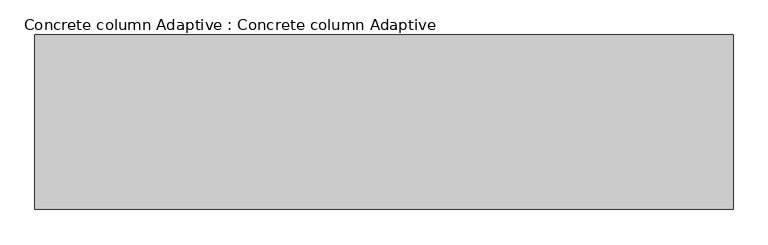
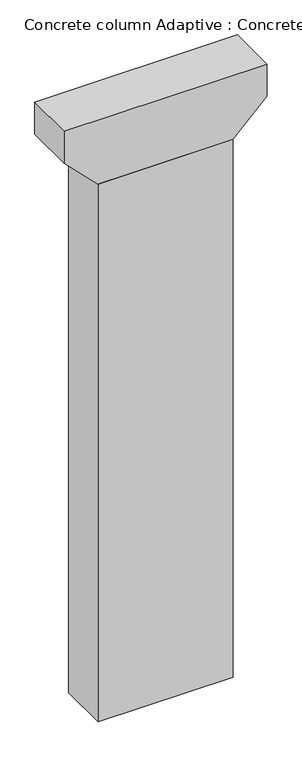
"""IFC4 building model written with IfcOpenShell, lengths in millimetres: proxy geometry, Concrete column Adaptive : Concrete column Adaptive."""

import ifcopenshell
import ifcopenshell.guid

model = None  # the IFC model being written
_history = None  # IfcOwnerHistory: only IFC2X3 demands one
_inside = {}  # id of a spatial element -> (the spatial element, [elements in it])
_under = {}  # id of a project, library or spatial element -> (it, [spatial elements below it])
_declared = {}  # id of a project -> (the project, [libraries it declares])
_typed = {}  # id of a type object -> (the type object, [elements of that type])
_made_of = {}  # id of a material, layer set ... -> (it, [elements and type objects made of it])


def new_model(schema):
    """Start an empty IFC model of exactly this schema.

    Asked for "IFC4X3", IfcOpenShell would pick the latest addendum, in which some entities
    have other attributes; the version numbers below select the first issue.
    IFC2X3 requires an IfcOwnerHistory on every rooted entity: one is made here for all.
    """
    global model, _history
    if schema == "IFC4X3":
        model = ifcopenshell.file(schema_version=(4, 3, 0, 0))
    else:
        model = ifcopenshell.file(schema=schema)
    _inside.clear()
    _under.clear()
    _declared.clear()
    _typed.clear()
    _made_of.clear()
    _history = None
    if model.schema == "IFC2X3":
        org = make("IfcOrganization", Name="unknown")
        user = make(
            "IfcPersonAndOrganization",
            ThePerson=make("IfcPerson", FamilyName="unknown"),
            TheOrganization=org,
        )
        app = make(
            "IfcApplication",
            ApplicationDeveloper=org,
            Version="unknown",
            ApplicationFullName="unknown",
            ApplicationIdentifier="unknown",
        )
        _history = make(
            "IfcOwnerHistory",
            OwningUser=user,
            OwningApplication=app,
            ChangeAction="ADDED",
            CreationDate=0,
        )
    return model


def make(cls, **values):
    """One entity of the class cls with the attributes given. An attribute that is None is left unset."""
    return model.create_entity(
        cls, **{name: value for name, value in values.items() if value is not None}
    )


def rooted(cls, **values):
    """An entity with a GlobalId (a new one), such as an element, a storey or a relation."""
    return make(cls, GlobalId=ifcopenshell.guid.new(), OwnerHistory=_history, **values)


def si_unit(unit_type, name, prefix=None):
    """IfcSIUnit, for example si_unit("LENGTHUNIT", "METRE", prefix="MILLI")."""
    return make("IfcSIUnit", UnitType=unit_type, Prefix=prefix, Name=name)


def assignment(units):
    """IfcUnitAssignment: the units of a project."""
    return None if units is None else make("IfcUnitAssignment", Units=units)


def point(xyz):
    """IfcCartesianPoint."""
    return None if xyz is None else make("IfcCartesianPoint", Coordinates=xyz)


def direction(xyz):
    """IfcDirection."""
    return None if xyz is None else make("IfcDirection", DirectionRatios=xyz)


def frame(location, z_axis=None, x_axis=None):
    """IfcAxis2Placement3D, a coordinate frame: its origin and axes. An axis left out is left unset."""
    return make(
        "IfcAxis2Placement3D",
        Location=point(location),
        Axis=direction(z_axis),
        RefDirection=direction(x_axis),
    )


def origin():
    """The frame at (0, 0, 0) with its axes left unset."""
    return frame((0.0, 0.0, 0.0))


def origin_with_axes():
    """The frame at (0, 0, 0) with the z axis (0, 0, 1) and the x axis (1, 0, 0) written out."""
    return frame((0.0, 0.0, 0.0), z_axis=(0.0, 0.0, 1.0), x_axis=(1.0, 0.0, 0.0))


def place(relative_to, where):
    """IfcLocalPlacement: puts the frame where relative to a parent placement (None: the world)."""
    return make(
        "IfcLocalPlacement", PlacementRelTo=relative_to, RelativePlacement=where
    )


def context(
    kind, dimensions, precision=None, world=None, true_north=None, identifier=None
):
    """IfcGeometricRepresentationContext, for example the 3D "Model" context."""
    return make(
        "IfcGeometricRepresentationContext",
        ContextIdentifier=identifier,
        ContextType=kind,
        CoordinateSpaceDimension=dimensions,
        Precision=precision,
        WorldCoordinateSystem=world,
        TrueNorth=true_north,
    )


def project(units=None, contexts=None):
    """IfcProject with its units and contexts."""
    return rooted(
        "IfcProject",
        Name="project",
        RepresentationContexts=contexts,
        UnitsInContext=assignment(units),
    )


def spatial(cls, under=None, at=None, **own):
    """A site, building, storey or space (cls), placed at a placement, below another one or the project."""
    s = rooted(cls, ObjectPlacement=at, **own)
    if under is not None:
        _under.setdefault(under.id(), (under, []))[1].append(s)
    return s


def polyline(points):
    """IfcPolyline through the points."""
    return make("IfcPolyline", Points=[point(p) for p in points])


def outline(outer, holes=None, kind="AREA"):
    """IfcArbitraryClosedProfileDef: a profile drawn as a closed curve; with holes, ...WithVoids."""
    if holes is None:
        return make("IfcArbitraryClosedProfileDef", ProfileType=kind, OuterCurve=outer)
    return make(
        "IfcArbitraryProfileDefWithVoids",
        ProfileType=kind,
        OuterCurve=outer,
        InnerCurves=holes,
    )


def extrude(swept, where, along, depth):
    """IfcExtrudedAreaSolid: the profile swept, set in the frame where, extruded along a direction by depth."""
    return make(
        "IfcExtrudedAreaSolid",
        SweptArea=swept,
        Position=where,
        ExtrudedDirection=direction(along),
        Depth=depth,
    )


def shape(context_of_items, identifier, shape_type, items):
    """IfcShapeRepresentation: the items that make up one representation, for example the "Body"."""
    return make(
        "IfcShapeRepresentation",
        ContextOfItems=context_of_items,
        RepresentationIdentifier=identifier,
        RepresentationType=shape_type,
        Items=items,
    )


def source(mapping_origin, context_of_items, identifier, shape_type, items):
    """IfcRepresentationMap: a shape defined once, which mapped items show again and again."""
    return make(
        "IfcRepresentationMap",
        MappingOrigin=mapping_origin,
        MappedRepresentation=shape(context_of_items, identifier, shape_type, items),
    )


def transform(
    local_origin,
    x_axis=None,
    y_axis=None,
    z_axis=None,
    scale=None,
    scale2=None,
    scale3=None,
    uniform=True,
):
    """IfcCartesianTransformationOperator3D, or its non-uniform kind. x_axis, y_axis, z_axis: its Axis1, 2, 3."""
    if uniform:
        return make(
            "IfcCartesianTransformationOperator3D",
            Axis1=direction(x_axis),
            Axis2=direction(y_axis),
            LocalOrigin=point(local_origin),
            Scale=scale,
            Axis3=direction(z_axis),
        )
    return make(
        "IfcCartesianTransformationOperator3DnonUniform",
        Axis1=direction(x_axis),
        Axis2=direction(y_axis),
        LocalOrigin=point(local_origin),
        Scale=scale,
        Axis3=direction(z_axis),
        Scale2=scale2,
        Scale3=scale3,
    )


def mapped(mapping_source, mapping_target):
    """IfcMappedItem: shows the shape of a source again, moved by a transform."""
    return make(
        "IfcMappedItem", MappingSource=mapping_source, MappingTarget=mapping_target
    )


def made_of(thing, what):
    """Note that an element or type object is made of a material, layer set ...; save() writes the relation."""
    if what is not None:
        _made_of.setdefault(what.id(), (what, []))[1].append(thing)
    return thing


def element(
    cls,
    number,
    at=None,
    inside=None,
    cuts=None,
    type_object=None,
    material=None,
    context=None,
    identifier="Body",
    shape_type=None,
    held_by="IfcProductDefinitionShape",
    body=None,
    shapes=None,
    **own,
):
    """One element of the class cls, such as IfcWall. Its Tag is "e" and its number.

    at: its placement. inside: the storey or other place that contains it. cuts: it is an
    opening in that element (IfcRelVoidsElement). A single representation is given by context,
    identifier, shape_type and body (its items); several are given by shapes. held_by: the class
    of the entity that holds the representations. save() writes the other relations.
    """
    e = rooted(cls, Tag="e%d" % number, ObjectPlacement=at, **own)
    if body is not None:
        shapes = [shape(context, identifier, shape_type, body)]
    if shapes is not None:
        e.Representation = make(held_by, Representations=shapes)
    if inside is not None:
        _inside.setdefault(inside.id(), (inside, []))[1].append(e)
    if cuts is not None:
        rooted(
            "IfcRelVoidsElement", RelatingBuildingElement=cuts, RelatedOpeningElement=e
        )
    if type_object is not None:
        _typed.setdefault(type_object.id(), (type_object, []))[1].append(e)
    return made_of(e, material)


def aggregate(whole, parts):
    """IfcRelAggregates: a whole, such as a stair, and the parts it consists of."""
    return rooted("IfcRelAggregates", RelatingObject=whole, RelatedObjects=parts)


def save(model, path):
    """Write the relations noted so far, then the file.

    IfcRelAggregates (storeys below a building ...), IfcRelContainedInSpatialStructure (elements
    in a storey), IfcRelDefinesByType, IfcRelAssociatesMaterial and IfcRelDeclares: one each for
    every whole, place, type object, material and project.
    """
    for whole, parts in _under.values():
        aggregate(whole, parts)
    for where, things in _inside.values():
        rooted(
            "IfcRelContainedInSpatialStructure",
            RelatedElements=things,
            RelatingStructure=where,
        )
    for kind, things in _typed.values():
        rooted("IfcRelDefinesByType", RelatedObjects=things, RelatingType=kind)
    for what, things in _made_of.values():
        rooted("IfcRelAssociatesMaterial", RelatedObjects=things, RelatingMaterial=what)
    for by, libraries in _declared.values():
        rooted("IfcRelDeclares", RelatingContext=by, RelatedDefinitions=libraries)
    model.write(path)


def concrete_column_adaptive_concrete_column_adaptive_f79cb2c7(model_context):
    return source(origin(), model_context, "Body", "SweptSolid", [
        extrude(outline(polyline([(37594.0, 6000.0), (37594.0, -6000.0), (35594.0, -6000.0), (33594.0, -4000.0), (33594.0, 4000.0), (35594.0, 6000.0), (37594.0, 6000.0)])), frame((0.0, -1500.0, 0.0), z_axis=(0.0, 1.0, 0.0), x_axis=(0.0, 0.0, 1.0)), (0.0, 0.0, 1.0), 3000.0),
        extrude(outline(polyline([(-4000.0, -1500.0), (-4000.0, 1500.0), (4000.0, 1500.0), (4000.0, -1500.0), (-4000.0, -1500.0)])), origin_with_axes(), (0.0, 0.0, 1.0), 33594.0),
    ])


if __name__ == "__main__":
    model = new_model("IFC4")
    model_context = context("Model", 3, world=origin())
    ifc_project = project(units=[si_unit("LENGTHUNIT", "METRE", prefix="MILLI")], contexts=[model_context])
    site = spatial("IfcSite", under=ifc_project)
    building = spatial("IfcBuilding", under=site)
    placement = place(None, origin())
    concrete_column_adaptive_concrete_column_adaptive_shape = concrete_column_adaptive_concrete_column_adaptive_f79cb2c7(model_context)
    element("IfcBuildingElementProxy", 1, Name="Concrete column Adaptive : Concrete column Adaptive", ObjectType="Concrete column Adaptive : Concrete column Adaptive", at=placement, inside=building, context=model_context, shape_type="MappedRepresentation", body=[
        mapped(concrete_column_adaptive_concrete_column_adaptive_shape, transform((0.0, 0.0, 0.0), x_axis=(1.0, 0.0, 0.0), y_axis=(0.0, 1.0, 0.0), z_axis=(0.0, 0.0, 1.0))),
    ])
    save(model, "model.ifc")

# Revit data of these elements
# Type "Concrete column Adaptive : Concrete column Adaptive"
#   Height [instance default] = 30000 mm
#   Default Elevation = 0
# Element 1 (IfcBuildingElementProxy, "Concrete column Adaptive : Concrete column Adaptive")
#   Height = 33594 mm
